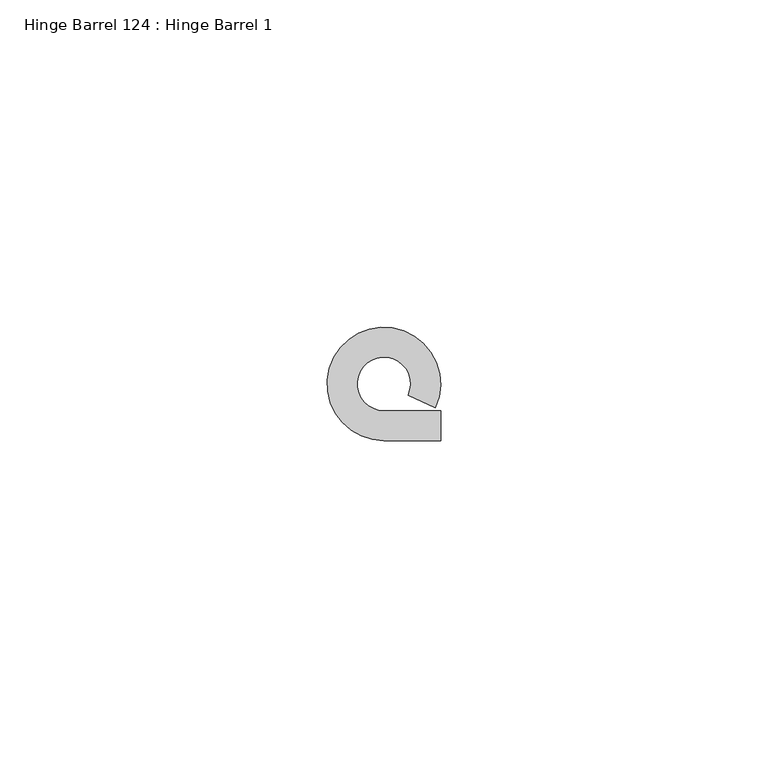
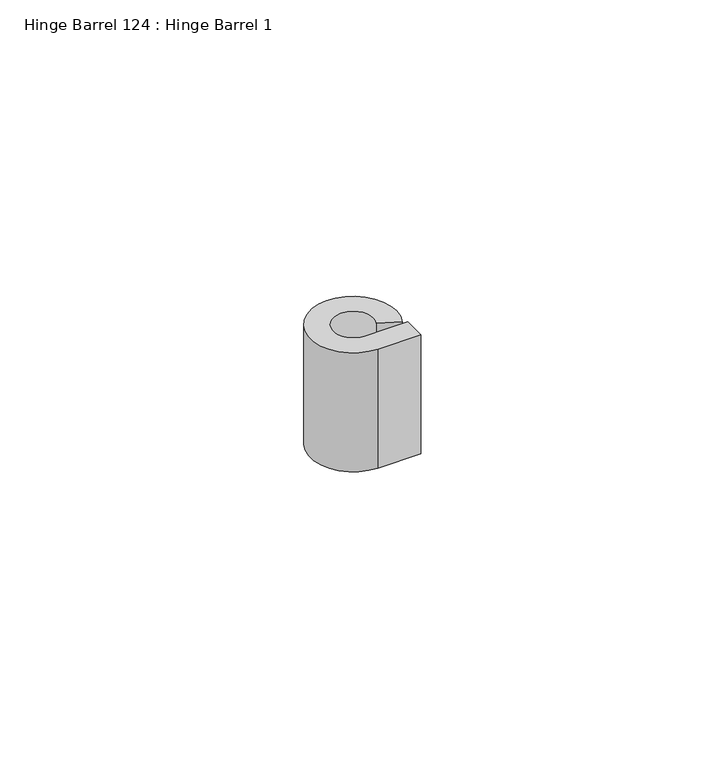
"""IFC4 building model written with IfcOpenShell, lengths in millimetres: proxy geometry, Hinge Barrel 124 : Hinge Barrel 1."""

from ifc_helpers import new_model, si_unit, point, frame, frame_2d, origin, place, context, project, spatial, polyline, circle_curve, trimmed, segment, composite_curve, outline, extrude, source, transform, mapped, element, save


def hinge_barrel_124_hinge_barrel_1_6a8bf010(model_context):
    return source(origin(), model_context, "Body", "SweptSolid", [
        extrude(outline(composite_curve([segment(polyline([(587323.2214739, -534104.7943841), (587327.7934739, -534104.7943841), (587327.7934739, -534109.3584466), (587319.1320739, -534109.3584466)]), True, "CONTINUOUS"), segment(trimmed(circle_curve(frame_2d((587319.1320739, -534100.7049841)), 8.6534625), [point((587319.1320739, -534109.3584466))], [point((587326.986084, -534104.3377433))], False, "CARTESIAN"), True, "CONTINUOUS"), segment(polyline([(587326.986084, -534104.3377433), (587322.8436736, -534102.421731)]), True, "CONTINUOUS"), segment(trimmed(circle_curve(frame_2d((587319.1320739, -534100.7049841)), 4.0894), [point((587322.8436736, -534102.421731))], [point((587319.1320739, -534104.7943841))], True, "CARTESIAN"), True, "CONTINUOUS"), segment(polyline([(587319.1320739, -534104.7943841), (587323.2214739, -534104.7943841)]), True, "CONTINUOUS")], self_intersect=False)), frame((0.0, 0.0, 1225.55), z_axis=(0.0, 0.0, 1.0), x_axis=(1.0, 0.0, 0.0)), (0.0, 0.0, 1.0), 25.4),
    ])


if __name__ == "__main__":
    model = new_model("IFC4")
    model_context = context("Model", 3, world=origin())
    ifc_project = project(units=[si_unit("LENGTHUNIT", "METRE", prefix="MILLI")], contexts=[model_context])
    site = spatial("IfcSite", under=ifc_project)
    building = spatial("IfcBuilding", under=site)
    placement = place(None, origin())
    hinge_barrel_124_hinge_barrel_1_shape = hinge_barrel_124_hinge_barrel_1_6a8bf010(model_context)
    element("IfcBuildingElementProxy", 1, Name="Hinge Barrel 124 : Hinge Barrel 1", ObjectType="Hinge Barrel 124 : Hinge Barrel 1", at=placement, inside=building, context=model_context, shape_type="MappedRepresentation", body=[
        mapped(hinge_barrel_124_hinge_barrel_1_shape, transform((0.0, 0.0, 0.0), x_axis=(1.0, 0.0, 0.0), y_axis=(0.0, 1.0, 0.0), z_axis=(0.0, 0.0, 1.0))),
    ])
    save(model, "model.ifc")

# Revit data of these elements
# Element 1 (IfcBuildingElementProxy, "Hinge Barrel 124 : Hinge Barrel 1")
#   Materials on its faces: "6\"X6\" WELD-ON STL BUTT HINGE"
# Materials
#   "6\"X6\" WELD-ON STL BUTT HINGE": class "Metal", colour RGB 189 187 185, transparency 0, Description = "Carbon steel", Cost = 0
